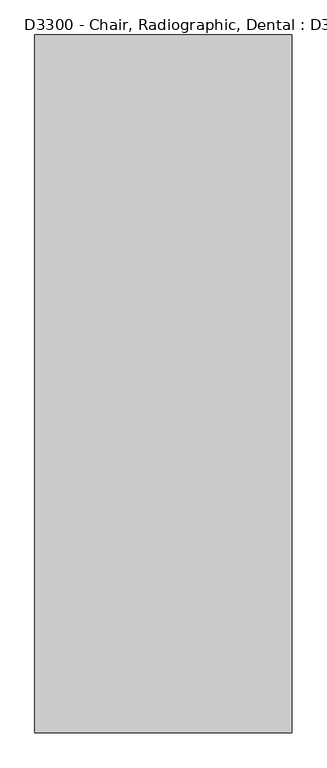
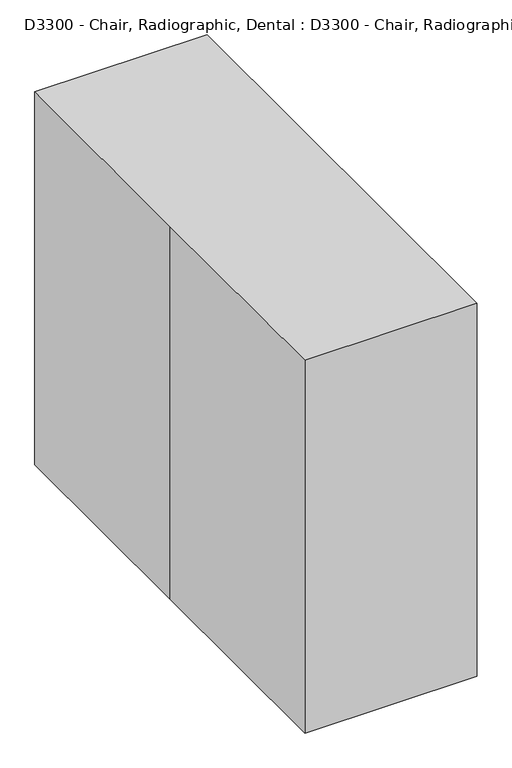
"""IFC4 building model written with IfcOpenShell, lengths in millimetres: proxy geometry, D3300 - Chair, Radiographic, Dental : D3300 - Chair, Radiographic, Dental."""

from ifc_helpers import new_model, si_unit, frame, origin, origin_with_axes, place, context, project, spatial, polyline, outline, extrude, source, transform, mapped, element, save


def d3300_chair_radiographic_dental_d3300_chair_radiographic_703e98a6(model_context):
    return source(origin(), model_context, "Body", "SweptSolid", [
        extrude(outline(polyline([(0.0, -31.75), (0.0, 0.0), (76.2, 0.0), (76.2, -31.75), (0.0, -31.75)])), frame((38.1, 382.0611467, 1179.3080235), z_axis=(0.0, 0.22495105434386323, 0.9743700647852357), x_axis=(-1.0, 0.0, 0.0)), (0.0, 0.0, 1.0), 82.55),
        extrude(outline(polyline([(0.0, -86.6214987), (0.0, 0.0), (304.8, 0.0), (304.8, -86.6214987), (0.0, -86.6214987)])), frame((153.6668582, 366.3045979, 1250.2004075), z_axis=(0.0, 0.22495105434386384, 0.9743700647852355), x_axis=(-1.0, 0.0, 0.0)), (0.0, 0.0, 1.0), 177.8),
        extrude(outline(polyline([(203.2, 914.4), (203.2, 609.6), (127.0, 609.6), (127.0, 838.2), (-203.2, 838.2), (-203.2, 914.4), (203.2, 914.4)])), frame((-292.7334291, 0.0, 0.0), z_axis=(1.0, 0.0, 0.0), x_axis=(0.0, 1.0, 0.0)), (0.0, 0.0, 1.0), 52.0668582),
        extrude(outline(polyline([(203.2, 914.4), (203.2, 609.6), (127.0, 609.6), (127.0, 838.2), (-203.2, 838.2), (-203.2, 914.4), (203.2, 914.4)])), frame((240.6665709, 0.0, 0.0), z_axis=(1.0, 0.0, 0.0), x_axis=(0.0, 1.0, 0.0)), (0.0, 0.0, 1.0), 55.7916128),
        extrude(outline(polyline([(-465.5789493, 83.7157526), (-664.2419881, 144.4531389), (-649.3895055, 193.0334205), (-532.0831721, 157.1692752), (-365.1888293, 703.0560737), (238.3220406, 703.0560737), (349.9832239, 1186.7137955), (445.0753191, 1164.7600555), (316.9065213, 609.6), (-304.8, 609.6), (-465.5789493, 83.7157526)])), frame((-240.6665709, 0.0, 0.0), z_axis=(1.0, 0.0, 0.0), x_axis=(0.0, 1.0, 0.0)), (0.0, 0.0, 1.0), 481.3331418),
        extrude(outline(polyline([(296.4581837, 304.8), (296.4581837, -304.8), (-292.7334291, -304.8), (-292.7334291, 304.8), (296.4581837, 304.8)])), origin_with_axes(), (0.0, 0.0, 1.0), 609.6),
        extrude(outline(polyline([(-355.6, 965.2), (355.6, 965.2), (355.6, -965.2), (-355.6, -965.2), (-355.6, 0.0), (-355.6, 965.2)])), origin_with_axes(), (0.0, 0.0, 1.0), 1625.6),
    ])


if __name__ == "__main__":
    model = new_model("IFC4")
    model_context = context("Model", 3, world=origin())
    ifc_project = project(units=[si_unit("LENGTHUNIT", "METRE", prefix="MILLI")], contexts=[model_context])
    site = spatial("IfcSite", under=ifc_project)
    building = spatial("IfcBuilding", under=site)
    placement = place(None, origin())
    d3300_chair_radiographic_dental_d3300_chair_radiographic_shape = d3300_chair_radiographic_dental_d3300_chair_radiographic_703e98a6(model_context)
    element("IfcBuildingElementProxy", 1, Name="D3300 - Chair, Radiographic, Dental : D3300 - Chair, Radiographic, Dental", ObjectType="D3300 - Chair, Radiographic, Dental : D3300 - Chair, Radiographic, Dental", at=placement, inside=building, context=model_context, shape_type="MappedRepresentation", body=[
        mapped(d3300_chair_radiographic_dental_d3300_chair_radiographic_shape, transform((0.0, 0.0, 0.0), x_axis=(1.0, 0.0, 0.0), y_axis=(0.0, 1.0, 0.0), z_axis=(0.0, 0.0, 1.0))),
    ])
    save(model, "model.ifc")

# Revit data of these elements
# Type "D3300 - Chair, Radiographic, Dental : D3300 - Chair, Radiographic, Dental"
#   Watts2 = "0"
#   Watts1 = "1440"
#   Unit_Issue = "EA"
#   UTIL_6_Misc = "-"
#   UTIL_5_NonMedGas = "-"
#   UTIL_4_MiscGas = "-"
#   UTIL_3_MedGas = "-"
#   UTIL_2_Elec = "A"
#   UTIL_1_WaterDrain = "-"
#   Nomenclature = "Chair, Radiographic, Dental"
#   NSN = "6520"
#   Location [instance default] = ""
#   JSN = "D3300"
#   Fund_Source_VA = "-"
#   Fund_Source_Navy = "-"
#   Fund_Source_Army = "-"
#   Fund_Source_AF = "-"
#   ELEC_Volts2 = "0"
#   ELEC_Volts1 = "120"
#   ELEC_Phase2 = "0"
#   ELEC_Phase1 = "1"
#   ELEC_HertzSwitch = "0"
#   ELEC_HertzDependent = "-1"
#   ELEC_Hertz = "60"
#   ELEC_Amps2 = "0"
#   ELEC_Amps1 = "12"
#   DetailDescription = "Dental x-ray chair. This chair is used in intraoral dental radiography and can be used as any dental chair, and is equipped with adjustable height capability. Standard dental operatory chairs can be used for this purpose and may enhance clinical uniformity. Specify color at time of ordering."
#   CAT_VA = "C"
#   CAT_Navy = "C"
#   CAT_IHS = "-"
#   CAT_Army = "C"
#   CAT_AF = "C"
#   BTUperhour = "0"
#   Weight_IP = 280
#   DIM_Width_IP = 2' - 4"
#   DIM_Height_IP = 5' - 4"
#   DIM_Depth_IP = 6' - 4"
# Element 1 (IfcBuildingElementProxy, "D3300 - Chair, Radiographic, Dental : D3300 - Chair, Radiographic, Dental")
#   Location = "DNXS1"
#   Materials on its faces: "EquipSpace"
# Materials
#   "EquipSpace": class "Unassigned", colour RGB 221 217 195, transparency 0.5
